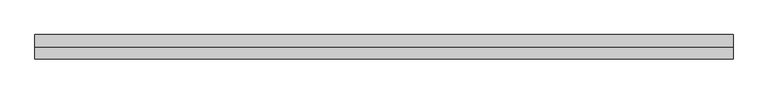
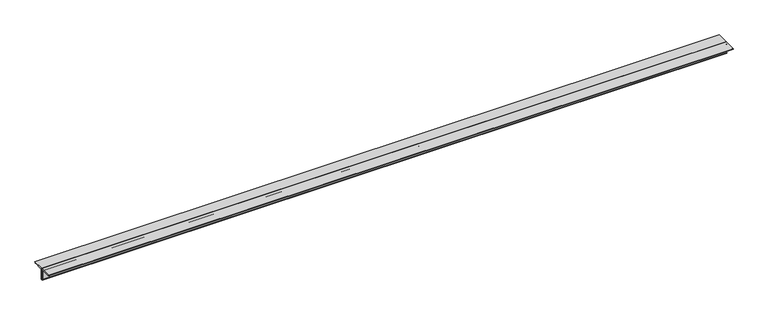
"""IFC4 building model written with IfcOpenShell, lengths in millimetres: member geometry, Steel Framing_2Ls_KS : H_SB_AR_S02_2Ls-100x100x10_VBR1."""

from ifc_helpers import new_model, si_unit, point, frame, frame_2d, origin, place, context, project, spatial, polyline, circle_curve, trimmed, segment, composite_curve, outline, extrude, source, transform, mapped, element, save


def member_66534584(model_context):
    return source(origin(), model_context, "Body", "SweptSolid", [
        extrude(outline(composite_curve([segment(polyline([(0.0, 28.2), (100.0, 28.2)]), True, "CONTINUOUS"), segment(trimmed(circle_curve(frame_2d((90.0, 28.2)), 10.0), [point((100.0, 28.2))], [point((90.0, 18.2))], False, "CARTESIAN"), True, "CONTINUOUS"), segment(polyline([(90.0, 18.2), (20.0, 18.2)]), True, "CONTINUOUS"), segment(trimmed(circle_curve(frame_2d((20.0, 8.2)), 10.0), [point((20.0, 18.2))], [point((10.0, 8.2))], True, "CARTESIAN"), True, "CONTINUOUS"), segment(polyline([(10.0, 8.2), (10.0, -61.8)]), True, "CONTINUOUS"), segment(trimmed(circle_curve(frame_2d((0.0, -61.8)), 10.0), [point((10.0, -61.8))], [point((0.0, -71.8))], False, "CARTESIAN"), True, "CONTINUOUS"), segment(polyline([(0.0, -71.8), (0.0, 28.2)]), True, "CONTINUOUS")], self_intersect=False)), frame((-2842.7759474, 0.0, 0.0), z_axis=(1.0, 0.0, 0.0), x_axis=(0.0, 1.0, 0.0)), (0.0, 0.0, 1.0), 5681.2399254),
        extrude(outline(composite_curve([segment(polyline([(0.0, 28.2), (0.0, -71.8)]), True, "CONTINUOUS"), segment(trimmed(circle_curve(frame_2d((0.0, -61.8)), 10.0), [point((0.0, -71.8))], [point((-10.0, -61.8))], False, "CARTESIAN"), True, "CONTINUOUS"), segment(polyline([(-10.0, -61.8), (-10.0, 8.2)]), True, "CONTINUOUS"), segment(trimmed(circle_curve(frame_2d((-20.0, 8.2)), 10.0), [point((-10.0, 8.2))], [point((-20.0, 18.2))], True, "CARTESIAN"), True, "CONTINUOUS"), segment(polyline([(-20.0, 18.2), (-90.0, 18.2)]), True, "CONTINUOUS"), segment(trimmed(circle_curve(frame_2d((-90.0, 28.2)), 10.0), [point((-90.0, 18.2))], [point((-100.0, 28.2))], False, "CARTESIAN"), True, "CONTINUOUS"), segment(polyline([(-100.0, 28.2), (0.0, 28.2)]), True, "CONTINUOUS")], self_intersect=False)), frame((-2842.7759474, 0.0, 0.0), z_axis=(1.0, 0.0, 0.0), x_axis=(0.0, 1.0, 0.0)), (0.0, 0.0, 1.0), 5681.2399254),
    ])


if __name__ == "__main__":
    model = new_model("IFC4")
    model_context = context("Model", 3, world=origin())
    ifc_project = project(units=[si_unit("LENGTHUNIT", "METRE", prefix="MILLI")], contexts=[model_context])
    site = spatial("IfcSite", under=ifc_project)
    building = spatial("IfcBuilding", under=site)
    placement = place(None, origin())
    member_shape = member_66534584(model_context)
    element("IfcMember", 1, ObjectType="Steel Framing_2Ls_KS : H_SB_AR_S02_2Ls-100x100x10_VBR1", at=placement, inside=building, context=model_context, shape_type="MappedRepresentation", body=[
        mapped(member_shape, transform((0.0, 0.0, 0.0), x_axis=(1.0, 0.0, 0.0), y_axis=(0.0, 1.0, 0.0), z_axis=(0.0, 0.0, 1.0))),
    ])
    save(model, "model.ifc")

# Revit data of these elements
# Type "Steel Framing_2Ls_KS : H_SB_AR_S02_2Ls-100x100x10_VBR1"
#   Type Comments = "MAIN"
#   Type Mark = "VBR1"
#   H_SectionID = "2Ls-100x100x10"
#   Assembly Code = "B10"
#   Legs = "LLBB"
#   H_Ratio for Additional Steel Plate = 0.2
#   W = 0
#   Perimeter = 0.80 m²/m
#   Nominal Weight = 29.80 kgf/m
#   Length [instance default] = 1524 mm
#   Space = 0 mm
#   b = 100 mm
#   d = 100 mm
#   t = 10 mm
#   y = 28.2 mm
#   A = 0.0038 m²
#   Structural Material [instance default] = Steel, 45-345
# Element 1 (IfcMember, "Steel Framing_2Ls_KS : H_SB_AR_S02_2Ls-100x100x10_VBR1")
#   Materials on its faces: "Steel, 45-345"
# Materials
#   "Steel, 45-345": class "Metal", colour RGB 189 187 185, transparency 0, Description = "Steel 345 MPa", Cost = 0
